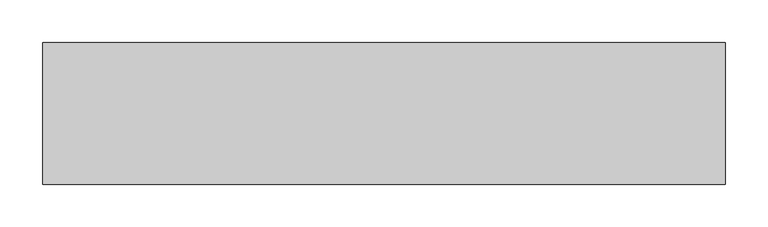
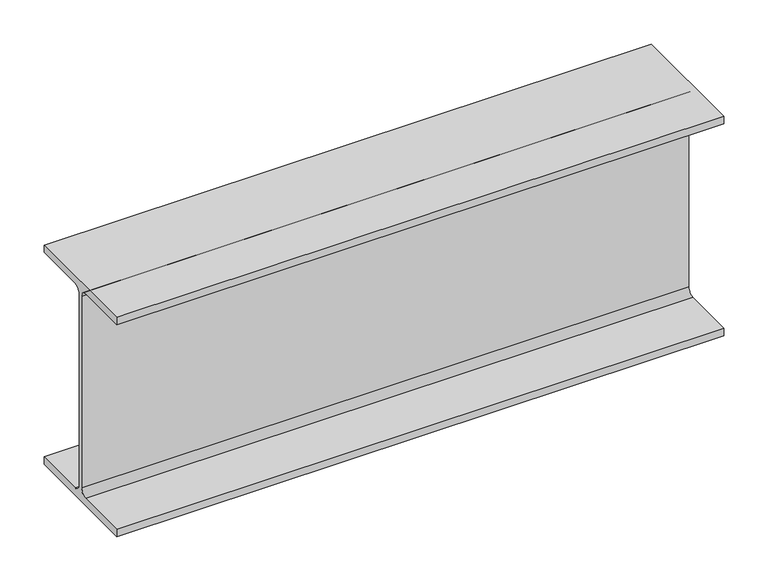
"""IFC4 building model written with IfcOpenShell, lengths in millimetres: beam geometry, Old_Steel Beam_H-KSD3502 : H_SB_ASB_H-300×150x6.5x9."""

from ifc_helpers import new_model, si_unit, point, frame, frame_2d, origin, place, context, project, spatial, polyline, circle_curve, trimmed, segment, composite_curve, outline, extrude, source, transform, mapped, element, save


def beam_f019c22a(model_context):
    return source(origin(), model_context, "Body", "SweptSolid", [
        extrude(outline(composite_curve([segment(polyline([(82.5, -141.5), (82.5, -151.7), (-82.5, -151.7), (-82.5, -141.5), (-11.9, -141.5)]), True, "CONTINUOUS"), segment(trimmed(circle_curve(frame_2d((-11.9, -132.6)), 8.9), [point((-11.9, -141.5))], [point((-3.0, -132.6))], True, "CARTESIAN"), True, "CONTINUOUS"), segment(polyline([(-3.0, -132.6), (-3.0, 132.6)]), True, "CONTINUOUS"), segment(trimmed(circle_curve(frame_2d((-11.9, 132.6)), 8.9), [point((-3.0, 132.6))], [point((-11.9, 141.5))], True, "CARTESIAN"), True, "CONTINUOUS"), segment(polyline([(-11.9, 141.5), (-82.5, 141.5), (-82.5, 151.7), (82.5, 151.7), (82.5, 141.5), (11.9, 141.5)]), True, "CONTINUOUS"), segment(trimmed(circle_curve(frame_2d((11.9, 132.6)), 8.9), [point((11.9, 141.5))], [point((3.0, 132.6))], True, "CARTESIAN"), True, "CONTINUOUS"), segment(polyline([(3.0, 132.6), (3.0, -132.6)]), True, "CONTINUOUS"), segment(trimmed(circle_curve(frame_2d((11.9, -132.6)), 8.9), [point((3.0, -132.6))], [point((11.9, -141.5))], True, "CARTESIAN"), True, "CONTINUOUS"), segment(polyline([(11.9, -141.5), (82.5, -141.5)]), True, "CONTINUOUS")], self_intersect=False)), frame((-445.0, 0.0, 0.0), z_axis=(1.0, 0.0, 0.0), x_axis=(0.0, 1.0, 0.0)), (0.0, 0.0, 1.0), 794.8),
    ])


if __name__ == "__main__":
    model = new_model("IFC4")
    model_context = context("Model", 3, world=origin())
    ifc_project = project(units=[si_unit("LENGTHUNIT", "METRE", prefix="MILLI")], contexts=[model_context])
    site = spatial("IfcSite", under=ifc_project)
    building = spatial("IfcBuilding", under=site)
    placement = place(None, origin())
    beam_shape = beam_f019c22a(model_context)
    element("IfcBeam", 1, ObjectType="Old_Steel Beam_H-KSD3502 : H_SB_ASB_H-300×150x6.5x9", at=placement, inside=building, context=model_context, shape_type="MappedRepresentation", body=[
        mapped(beam_shape, transform((0.0, 0.0, 0.0), x_axis=(1.0, 0.0, 0.0), y_axis=(0.0, 1.0, 0.0), z_axis=(0.0, 0.0, 1.0))),
    ])
    save(model, "model.ifc")

# Revit data of these elements
# Type "Old_Steel Beam_H-KSD3502 : H_SB_ASB_H-300×150x6.5x9"
#   Width = 15.0 cm
#   Web Thickness = 0.65 cm
#   Web Fillet = 1.3 cm
#   Warping Constant = 107174.0 cm⁶
#   Torsional Moment of Inertia = 9.9539 cm⁴
#   Torsional Modulus = 1.0 cm³
#   Section Area = 46.78 cm²
#   Plastic Modulus weak axis = 105.0 cm³
#   Plastic Modulus strong axis = 542.0 cm³
#   Perimeter = 1.17 m²/m
#   Nominal Weight = 36.70 kgf/m
#   Moment of Inertia weak axis = 508.00 cm⁴
#   Moment of Inertia strong axis = 7210.00 cm⁴
#   Height = 30.0 cm
#   Flange Thickness = 0.9 cm
#   Elastic Modulus weak axis = 67.7 cm³
#   Elastic Modulus strong axis = 481.0 cm³
#   Centroid Vertical = 15.0 cm
#   Centroid Horizontal = 7.5 cm
#   Length [instance default] = 1.5240 m
#   Structural Material [instance default] = Steel, 45-345
#   Assembly Code = ""
# Element 1 (IfcBeam, "Old_Steel Beam_H-KSD3502 : H_SB_ASB_H-300×150x6.5x9")
#   Structural Material = none
# Materials
#   "Steel, 45-345": class "Metal", colour RGB 189 187 185, transparency 0, Description = "Steel 345 MPa", Cost = 0
